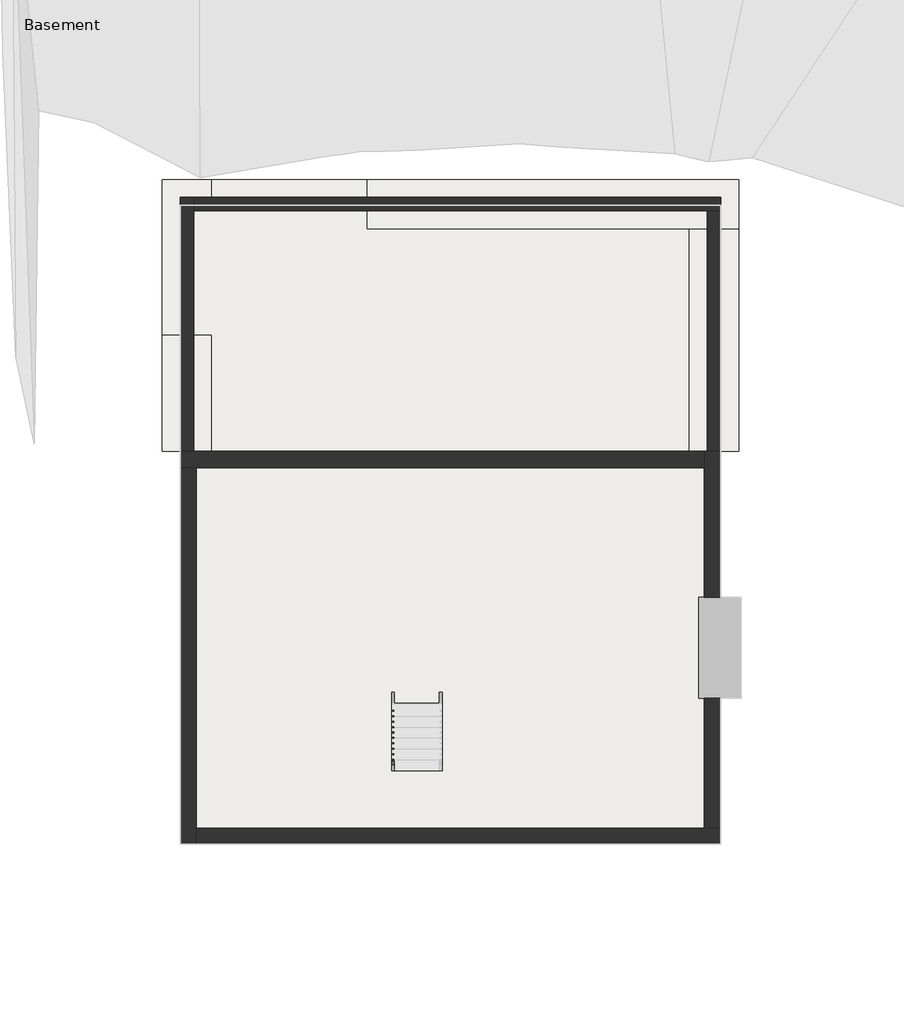
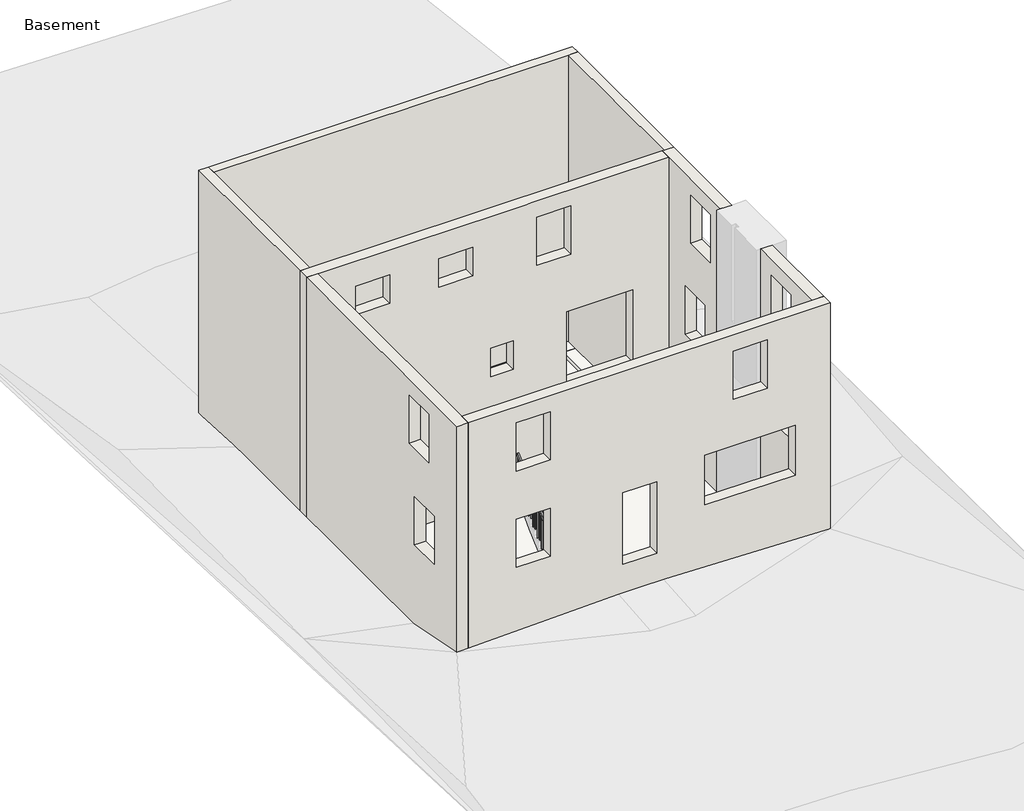
# One storey, part 1 of 2: 8 walls, 3 footings, 2 slabs, 1 railing.
"""IFC4 building model written with IfcOpenShell, lengths in millimetres."""

from ifc_helpers import new_model, si_unit, frame, origin, place, context, project, spatial, polyline, outline, extrude, faceted_brep, element, save

model = new_model("IFC4")

# Units and contexts
model_context = context("Model", 3, world=origin())
ifc_project = project(units=[si_unit("LENGTHUNIT", "METRE", prefix="MILLI")], contexts=[model_context])

# Site, building, storey
site = spatial("IfcSite", under=ifc_project)
building = spatial("IfcBuilding", under=site)
storey = spatial("IfcBuildingStorey", under=building, Name="Basement", Elevation=-2667.0)

# Footings
placement = place(None, origin())
element("IfcFooting", 1, ObjectType="Bearing Footing - 36\" x 12\"", at=placement, inside=storey, context=model_context, shape_type="Brep", body=[
    faceted_brep([(-5404.9803068, 3152.0888758, -2667.0), (-6319.3803068, 3152.0888758, -2667.0), (-6319.3803068, 3152.0888758, -2971.8), (-5404.9803068, 3152.0888758, -2971.8), (-6319.3803068, 5311.0888758, -2667.0), (-5404.9803068, 5311.0888758, -2667.0), (-5404.9803068, 5311.0888758, -2971.8), (-6319.3803068, 5311.0888758, -2971.8)], [[[0, 1, 2, 3]], [[4, 5, 6, 7]], [[0, 5, 4, 1]], [[2, 1, 4, 7]], [[3, 2, 7, 6]], [[0, 3, 6, 5]]]),
    faceted_brep([(-5404.9803068, 5311.0888758, -3124.2), (-6319.3803068, 5311.0888758, -3124.2), (-6319.3803068, 5311.0888758, -3429.0), (-5404.9803068, 5311.0888758, -3429.0), (-5404.9803068, 7292.2888758, -3124.2), (-5404.9803068, 8206.6888758, -3124.2), (-6319.3803068, 8206.6888758, -3124.2), (-6319.3803068, 8206.6888758, -3429.0), (-5404.9803068, 8206.6888758, -3429.0), (-5404.9803068, 7292.2888758, -3429.0)], [[[0, 1, 2, 3]], [[0, 4, 5, 6, 1]], [[2, 1, 6, 7]], [[3, 2, 7, 8, 9]], [[0, 3, 9, 8, 5, 4]], [[6, 5, 8, 7]]]),
])
element("IfcFooting", 2, ObjectType="Bearing Footing - 36\" x 12\"", at=placement, inside=storey, context=model_context, shape_type="Brep", body=[
    faceted_brep([(-2509.3803068, 8206.6888758, -3429.0), (-2509.3803068, 8206.6888758, -3124.2), (-2509.3803068, 7292.2888758, -3124.2), (-2509.3803068, 7292.2888758, -3429.0), (-5404.9803068, 8206.6888758, -3124.2), (-5404.9803068, 7292.2888758, -3124.2), (-5404.9803068, 8206.6888758, -3429.0), (-5404.9803068, 7292.2888758, -3429.0)], [[[0, 1, 2, 3]], [[2, 1, 4, 5]], [[1, 0, 6, 4]], [[0, 3, 7, 6]], [[3, 2, 5, 7]], [[5, 4, 6, 7]]]),
    faceted_brep([(-2509.3803068, 8206.6888758, -2667.0), (-2509.3803068, 8206.6888758, -2971.8), (-2509.3803068, 7292.2888758, -2971.8), (-2509.3803068, 7292.2888758, -2667.0), (4399.4196932, 8206.6888758, -2667.0), (3485.0196932, 7292.2888758, -2667.0), (4399.4196932, 7292.2888758, -2667.0), (4399.4196932, 8206.6888758, -2971.8), (4399.4196932, 7292.2888758, -2971.8), (3485.0196932, 7292.2888758, -2971.8)], [[[0, 1, 2, 3]], [[4, 0, 3, 5, 6]], [[1, 0, 4, 7]], [[2, 1, 7, 8, 9]], [[3, 2, 9, 8, 6, 5]], [[4, 6, 8, 7]]]),
])
element("IfcFooting", 3, ObjectType="Bearing Footing - 36\" x 12\"", at=placement, inside=storey, context=model_context, shape_type="SweptSolid", body=[
    extrude(outline(polyline([(4399.4196932, 3152.0888758), (3485.0196932, 3152.0888758), (3485.0196932, 7292.2888758), (4399.4196932, 7292.2888758), (4399.4196932, 3152.0888758)])), frame((0.0, 0.0, -2971.8), z_axis=(0.0, 0.0, 1.0), x_axis=(1.0, 0.0, 0.0)), (0.0, 0.0, 1.0), 304.8),
])

# Railing
element("IfcRailing", 4, ObjectType="Handrail - Rectangular", at=placement, inside=storey, context=model_context, shape_type="SweptSolid", body=[
    extrude(outline(polyline([(-2791.5111242, -1631.7331862), (-2791.5111242, -1562.1), (-149.9111242, 914.4), (-149.9111242, 844.7668138), (-2791.5111242, -1631.7331862)])), frame((-2052.1803068, 0.0, 0.0), z_axis=(1.0, 0.0, 0.0), x_axis=(0.0, 1.0, 0.0)), (0.0, 0.0, 1.0), 50.8),
    extrude(outline(polyline([(-241.9861242, 758.4465013), (-241.9861242, -190.5), (-261.0361242, -190.5), (-261.0361242, 740.5871263), (-241.9861242, 758.4465013)])), frame((-2036.3053068, 0.0, 0.0), z_axis=(1.0, 0.0, 0.0), x_axis=(0.0, 1.0, 0.0)), (0.0, 0.0, 1.0), 19.05),
    extrude(outline(polyline([(-343.5861242, 663.1965013), (-343.5861242, -190.5), (-362.6361242, -190.5), (-362.6361242, 645.3371263), (-343.5861242, 663.1965013)])), frame((-2036.3053068, 0.0, 0.0), z_axis=(1.0, 0.0, 0.0), x_axis=(0.0, 1.0, 0.0)), (0.0, 0.0, 1.0), 19.05),
    extrude(outline(polyline([(-445.1861242, 567.9465013), (-445.1861242, -381.0), (-464.2361242, -381.0), (-464.2361242, 550.0871263), (-445.1861242, 567.9465013)])), frame((-2036.3053068, 0.0, 0.0), z_axis=(1.0, 0.0, 0.0), x_axis=(0.0, 1.0, 0.0)), (0.0, 0.0, 1.0), 19.05),
    extrude(outline(polyline([(-546.7861242, 472.6965013), (-546.7861242, -381.0), (-565.8361242, -381.0), (-565.8361242, 454.8371263), (-546.7861242, 472.6965013)])), frame((-2036.3053068, 0.0, 0.0), z_axis=(1.0, 0.0, 0.0), x_axis=(0.0, 1.0, 0.0)), (0.0, 0.0, 1.0), 19.05),
    extrude(outline(polyline([(-648.3861242, 377.4465013), (-648.3861242, -571.5), (-667.4361242, -571.5), (-667.4361242, 359.5871263), (-648.3861242, 377.4465013)])), frame((-2036.3053068, 0.0, 0.0), z_axis=(1.0, 0.0, 0.0), x_axis=(0.0, 1.0, 0.0)), (0.0, 0.0, 1.0), 19.05),
    extrude(outline(polyline([(-749.9861242, 282.1965013), (-749.9861242, -571.5), (-769.0361242, -571.5), (-769.0361242, 264.3371263), (-749.9861242, 282.1965013)])), frame((-2036.3053068, 0.0, 0.0), z_axis=(1.0, 0.0, 0.0), x_axis=(0.0, 1.0, 0.0)), (0.0, 0.0, 1.0), 19.05),
    extrude(outline(polyline([(-851.5861242, 186.9465013), (-851.5861242, -762.0), (-870.6361242, -762.0), (-870.6361242, 169.0871263), (-851.5861242, 186.9465013)])), frame((-2036.3053068, 0.0, 0.0), z_axis=(1.0, 0.0, 0.0), x_axis=(0.0, 1.0, 0.0)), (0.0, 0.0, 1.0), 19.05),
    extrude(outline(polyline([(-953.1861242, 91.6965013), (-953.1861242, -762.0), (-972.2361242, -762.0), (-972.2361242, 73.8371263), (-953.1861242, 91.6965013)])), frame((-2036.3053068, 0.0, 0.0), z_axis=(1.0, 0.0, 0.0), x_axis=(0.0, 1.0, 0.0)), (0.0, 0.0, 1.0), 19.05),
    extrude(outline(polyline([(-1054.7861242, -3.5534987), (-1054.7861242, -952.5), (-1073.8361242, -952.5), (-1073.8361242, -21.4128737), (-1054.7861242, -3.5534987)])), frame((-2036.3053068, 0.0, 0.0), z_axis=(1.0, 0.0, 0.0), x_axis=(0.0, 1.0, 0.0)), (0.0, 0.0, 1.0), 19.05),
    extrude(outline(polyline([(-1156.3861242, -98.8034987), (-1156.3861242, -952.5), (-1175.4361242, -952.5), (-1175.4361242, -116.6628737), (-1156.3861242, -98.8034987)])), frame((-2036.3053068, 0.0, 0.0), z_axis=(1.0, 0.0, 0.0), x_axis=(0.0, 1.0, 0.0)), (0.0, 0.0, 1.0), 19.05),
    extrude(outline(polyline([(-1257.9861242, -194.0534987), (-1257.9861242, -1143.0), (-1277.0361242, -1143.0), (-1277.0361242, -211.9128737), (-1257.9861242, -194.0534987)])), frame((-2036.3053068, 0.0, 0.0), z_axis=(1.0, 0.0, 0.0), x_axis=(0.0, 1.0, 0.0)), (0.0, 0.0, 1.0), 19.05),
    extrude(outline(polyline([(-1359.5861242, -289.3034987), (-1359.5861242, -1143.0), (-1378.6361242, -1143.0), (-1378.6361242, -307.1628737), (-1359.5861242, -289.3034987)])), frame((-2036.3053068, 0.0, 0.0), z_axis=(1.0, 0.0, 0.0), x_axis=(0.0, 1.0, 0.0)), (0.0, 0.0, 1.0), 19.05),
    extrude(outline(polyline([(-1461.1861242, -384.5534987), (-1461.1861242, -1333.5), (-1480.2361242, -1333.5), (-1480.2361242, -402.4128737), (-1461.1861242, -384.5534987)])), frame((-2036.3053068, 0.0, 0.0), z_axis=(1.0, 0.0, 0.0), x_axis=(0.0, 1.0, 0.0)), (0.0, 0.0, 1.0), 19.05),
    extrude(outline(polyline([(-1562.7861242, -479.8034987), (-1562.7861242, -1333.5), (-1581.8361242, -1333.5), (-1581.8361242, -497.6628737), (-1562.7861242, -479.8034987)])), frame((-2036.3053068, 0.0, 0.0), z_axis=(1.0, 0.0, 0.0), x_axis=(0.0, 1.0, 0.0)), (0.0, 0.0, 1.0), 19.05),
    extrude(outline(polyline([(-1664.3861242, -575.0534987), (-1664.3861242, -1524.0), (-1683.4361242, -1524.0), (-1683.4361242, -592.9128737), (-1664.3861242, -575.0534987)])), frame((-2036.3053068, 0.0, 0.0), z_axis=(1.0, 0.0, 0.0), x_axis=(0.0, 1.0, 0.0)), (0.0, 0.0, 1.0), 19.05),
    extrude(outline(polyline([(-1765.9861242, -670.3034987), (-1765.9861242, -1524.0), (-1785.0361242, -1524.0), (-1785.0361242, -688.1628737), (-1765.9861242, -670.3034987)])), frame((-2036.3053068, 0.0, 0.0), z_axis=(1.0, 0.0, 0.0), x_axis=(0.0, 1.0, 0.0)), (0.0, 0.0, 1.0), 19.05),
    extrude(outline(polyline([(-1867.5861242, -765.5534987), (-1867.5861242, -1714.5), (-1886.6361242, -1714.5), (-1886.6361242, -783.4128737), (-1867.5861242, -765.5534987)])), frame((-2036.3053068, 0.0, 0.0), z_axis=(1.0, 0.0, 0.0), x_axis=(0.0, 1.0, 0.0)), (0.0, 0.0, 1.0), 19.05),
    extrude(outline(polyline([(-1969.1861242, -860.8034987), (-1969.1861242, -1714.5), (-1988.2361242, -1714.5), (-1988.2361242, -878.6628737), (-1969.1861242, -860.8034987)])), frame((-2036.3053068, 0.0, 0.0), z_axis=(1.0, 0.0, 0.0), x_axis=(0.0, 1.0, 0.0)), (0.0, 0.0, 1.0), 19.05),
    extrude(outline(polyline([(-2070.7861242, -956.0534987), (-2070.7861242, -1905.0), (-2089.8361242, -1905.0), (-2089.8361242, -973.9128737), (-2070.7861242, -956.0534987)])), frame((-2036.3053068, 0.0, 0.0), z_axis=(1.0, 0.0, 0.0), x_axis=(0.0, 1.0, 0.0)), (0.0, 0.0, 1.0), 19.05),
    extrude(outline(polyline([(-2172.3861242, -1051.3034987), (-2172.3861242, -1905.0), (-2191.4361242, -1905.0), (-2191.4361242, -1069.1628737), (-2172.3861242, -1051.3034987)])), frame((-2036.3053068, 0.0, 0.0), z_axis=(1.0, 0.0, 0.0), x_axis=(0.0, 1.0, 0.0)), (0.0, 0.0, 1.0), 19.05),
    extrude(outline(polyline([(-2273.9861242, -1146.5534987), (-2273.9861242, -2095.5), (-2293.0361242, -2095.5), (-2293.0361242, -1164.4128737), (-2273.9861242, -1146.5534987)])), frame((-2036.3053068, 0.0, 0.0), z_axis=(1.0, 0.0, 0.0), x_axis=(0.0, 1.0, 0.0)), (0.0, 0.0, 1.0), 19.05),
    extrude(outline(polyline([(-2375.5861242, -1241.8034987), (-2375.5861242, -2095.5), (-2394.6361242, -2095.5), (-2394.6361242, -1259.6628737), (-2375.5861242, -1241.8034987)])), frame((-2036.3053068, 0.0, 0.0), z_axis=(1.0, 0.0, 0.0), x_axis=(0.0, 1.0, 0.0)), (0.0, 0.0, 1.0), 19.05),
    extrude(outline(polyline([(-2477.1861242, -1337.0534987), (-2477.1861242, -2286.0), (-2496.2361242, -2286.0), (-2496.2361242, -1354.9128737), (-2477.1861242, -1337.0534987)])), frame((-2036.3053068, 0.0, 0.0), z_axis=(1.0, 0.0, 0.0), x_axis=(0.0, 1.0, 0.0)), (0.0, 0.0, 1.0), 19.05),
    extrude(outline(polyline([(-2578.7861242, -1432.3034987), (-2578.7861242, -2286.0), (-2597.8361242, -2286.0), (-2597.8361242, -1450.1628737), (-2578.7861242, -1432.3034987)])), frame((-2036.3053068, 0.0, 0.0), z_axis=(1.0, 0.0, 0.0), x_axis=(0.0, 1.0, 0.0)), (0.0, 0.0, 1.0), 19.05),
    extrude(outline(polyline([(-2680.3861242, -1527.5534987), (-2680.3861242, -2476.5), (-2699.4361242, -2476.5), (-2699.4361242, -1545.4128737), (-2680.3861242, -1527.5534987)])), frame((-2036.3053068, 0.0, 0.0), z_axis=(1.0, 0.0, 0.0), x_axis=(0.0, 1.0, 0.0)), (0.0, 0.0, 1.0), 19.05),
    extrude(outline(polyline([(-149.9111242, 844.7668138), (-149.9111242, -190.5), (-168.9611242, -190.5), (-168.9611242, 826.9074388), (-149.9111242, 844.7668138)])), frame((-2036.3053068, 0.0, 0.0), z_axis=(1.0, 0.0, 0.0), x_axis=(0.0, 1.0, 0.0)), (0.0, 0.0, 1.0), 19.05),
    extrude(outline(polyline([(-2772.4611242, -1613.8738112), (-2772.4611242, -2476.5), (-2791.5111242, -2476.5), (-2791.5111242, -1631.7331862), (-2772.4611242, -1613.8738112)])), frame((-2036.3053068, 0.0, 0.0), z_axis=(1.0, 0.0, 0.0), x_axis=(0.0, 1.0, 0.0)), (0.0, 0.0, 1.0), 19.05),
])

# Slabs
element("IfcSlab", 5, ObjectType="Pad 1", at=placement, inside=storey, context=model_context, shape_type="SweptSolid", body=[
    extrude(outline(polyline([(4069.2196932, 434.2888758), (4450.2196932, 434.2888758), (4450.2196932, -1445.3111242), (4069.2196932, -1445.3111242), (4069.2196932, -4163.1111242), (-5989.1803068, -4163.1111242), (-5989.1803068, 3152.0888758), (4069.2196932, 3152.0888758), (4069.2196932, 434.2888758)])), frame((0.0, 0.0, -3073.4), z_axis=(0.0, 0.0, 1.0), x_axis=(1.0, 0.0, 0.0)), (0.0, 0.0, 1.0), 304.8),
])
element("IfcSlab", 6, ObjectType="Pad 1", at=placement, inside=storey, context=model_context, shape_type="SweptSolid", body=[
    extrude(outline(polyline([(-5989.1803068, 7724.0888758), (4069.2196932, 7724.0888758), (4069.2196932, 3152.0888758), (-5989.1803068, 3152.0888758), (-5989.1803068, 7724.0888758)])), frame((0.0, 0.0, -3073.4), z_axis=(0.0, 0.0, 1.0), x_axis=(1.0, 0.0, 0.0)), (0.0, 0.0, 1.0), 304.8),
])

# Walls
element("IfcWall", 7, ObjectType="Generic - 10\"", at=placement, inside=storey, context=model_context, shape_type="Brep", body=[
    faceted_brep([(-5735.1803068, 3152.0888758, -2667.0), (-5735.1803068, 5311.0888758, -2667.0), (-5735.1803068, 5311.0888758, -3124.2), (-5735.1803068, 7622.4888758, -3124.2), (-5735.1803068, 7876.4888758, -3124.2), (-5735.1803068, 7876.4888758, 5486.4), (-5735.1803068, 7622.4888758, 5486.4), (-5735.1803068, 3152.0888758, 5486.4), (-5989.1803068, 3152.0888758, -2667.0), (-5989.1803068, 3152.0888758, 5486.4), (-5989.1803068, 7876.4888758, 5486.4), (-5989.1803068, 7876.4888758, -3124.2), (-5989.1803068, 5311.0888758, -3124.2), (-5989.1803068, 5311.0888758, -2667.0)], [[[0, 1, 2, 3, 4, 5, 6, 7]], [[8, 9, 10, 11, 12, 13]], [[1, 0, 8, 13]], [[2, 1, 13, 12]], [[4, 3, 2, 12, 11]], [[7, 6, 5, 10, 9]], [[5, 4, 11, 10]], [[0, 7, 9, 8]]]),
])
element("IfcWall", 8, ObjectType="Generic - 10\"", at=placement, inside=storey, context=model_context, shape_type="Brep", body=[
    faceted_brep([(-5735.1803068, 7622.4888758, -3124.2), (-2509.3803068, 7622.4888758, -3124.2), (-2509.3803068, 7622.4888758, -2667.0), (3815.2196932, 7622.4888758, -2667.0), (4069.2196932, 7622.4888758, -2667.0), (4069.2196932, 7622.4888758, 5486.4), (3815.2196932, 7622.4888758, 5486.4), (-5735.1803068, 7622.4888758, 5486.4), (-5735.1803068, 7876.4888758, -3124.2), (-5735.1803068, 7876.4888758, 5486.4), (4069.2196932, 7876.4888758, 5486.4), (4069.2196932, 7876.4888758, -2667.0), (-2509.3803068, 7876.4888758, -2667.0), (-2509.3803068, 7876.4888758, -3124.2)], [[[0, 1, 2, 3, 4, 5, 6, 7]], [[8, 9, 10, 11, 12, 13]], [[1, 0, 8, 13]], [[2, 1, 13, 12]], [[4, 3, 2, 12, 11]], [[7, 6, 5, 10, 9]], [[5, 4, 11, 10]], [[0, 7, 9, 8]]]),
])
element("IfcWall", 9, ObjectType="Generic - 10\"", at=placement, inside=storey, context=model_context, shape_type="SweptSolid", body=[
    extrude(outline(polyline([(3815.2196932, 3152.0888758), (3815.2196932, 7622.4888758), (4069.2196932, 7622.4888758), (4069.2196932, 3152.0888758), (3815.2196932, 3152.0888758)])), frame((0.0, 0.0, -2667.0), z_axis=(0.0, 0.0, 1.0), x_axis=(1.0, 0.0, 0.0)), (0.0, 0.0, 1.0), 8153.4),
])
element("IfcWall", 10, ObjectType="Generic - 12\"", at=placement, inside=storey, context=model_context, shape_type="Brep", body=[
    faceted_brep([(-5989.1803068, 2847.2888758, -2667.0), (-5684.3803068, 2847.2888758, -2667.0), (3764.4196932, 2847.2888758, -2667.0), (3764.4196932, 2847.2888758, 5486.4), (56.0196932, 2847.2888758, 5486.4), (-70.9803068, 2847.2888758, 5486.4), (-680.5803068, 2847.2888758, 5486.4), (-807.5803068, 2847.2888758, 5486.4), (-3169.7803068, 2847.2888758, 5486.4), (-3296.7803068, 2847.2888758, 5486.4), (-5684.3803068, 2847.2888758, 5486.4), (-5989.1803068, 2847.2888758, 5486.4), (1021.2196932, 2847.2888758, 0.0), (1021.2196932, 2847.2888758, 2057.4), (2799.2196932, 2847.2888758, 2057.4), (2799.2196932, 2847.2888758, 0.0), (-4160.3803068, 2847.2888758, 0.0), (-5023.9803068, 2847.2888758, 0.0), (-5023.9803068, 2847.2888758, 2032.0), (-4160.3803068, 2847.2888758, 2032.0), (-1036.1803068, 2847.2888758, 914.4), (-1036.1803068, 2847.2888758, 1727.2), (-426.5803068, 2847.2888758, 1727.2), (-426.5803068, 2847.2888758, 914.4), (-3919.0803068, 2847.2888758, 914.4), (-3919.0803068, 2847.2888758, 1727.2), (-3004.6803068, 2847.2888758, 1727.2), (-3004.6803068, 2847.2888758, 914.4), (208.4196932, 2847.2888758, 3657.6), (208.4196932, 2847.2888758, 5029.2), (1122.8196932, 2847.2888758, 5029.2), (1122.8196932, 2847.2888758, 3657.6), (-2433.1803068, 2847.2888758, 3962.4), (-2433.1803068, 2847.2888758, 4775.2), (-1518.7803068, 2847.2888758, 4775.2), (-1518.7803068, 2847.2888758, 3962.4), (-4668.3803068, 2847.2888758, 3962.4), (-4668.3803068, 2847.2888758, 4775.2), (-3753.9803068, 2847.2888758, 4775.2), (-3753.9803068, 2847.2888758, 3962.4), (3764.4196932, 3152.0888758, -2667.0), (-5989.1803068, 3152.0888758, -2667.0), (-5989.1803068, 3152.0888758, 5486.4), (3764.4196932, 3152.0888758, 5486.4), (1021.2196932, 3152.0888758, 2057.4), (1021.2196932, 3152.0888758, 0.0), (2799.2196932, 3152.0888758, 0.0), (2799.2196932, 3152.0888758, 2057.4), (-5023.9803068, 3152.0888758, 0.0), (-4160.3803068, 3152.0888758, 0.0), (-4160.3803068, 3152.0888758, 2032.0), (-5023.9803068, 3152.0888758, 2032.0), (-1036.1803068, 3152.0888758, 1727.2), (-1036.1803068, 3152.0888758, 914.4), (-426.5803068, 3152.0888758, 914.4), (-426.5803068, 3152.0888758, 1727.2), (-3919.0803068, 3152.0888758, 1727.2), (-3919.0803068, 3152.0888758, 914.4), (-3004.6803068, 3152.0888758, 914.4), (-3004.6803068, 3152.0888758, 1727.2), (208.4196932, 3152.0888758, 5029.2), (208.4196932, 3152.0888758, 3657.6), (1122.8196932, 3152.0888758, 3657.6), (1122.8196932, 3152.0888758, 5029.2), (-2433.1803068, 3152.0888758, 4775.2), (-2433.1803068, 3152.0888758, 3962.4), (-1518.7803068, 3152.0888758, 3962.4), (-1518.7803068, 3152.0888758, 4775.2), (-4668.3803068, 3152.0888758, 4775.2), (-4668.3803068, 3152.0888758, 3962.4), (-3753.9803068, 3152.0888758, 3962.4), (-3753.9803068, 3152.0888758, 4775.2)], [[[0, 1, 2, 3, 4, 5, 6, 7, 8, 9, 10, 11], [12, 13, 14, 15], [16, 17, 18, 19], [20, 21, 22, 23], [24, 25, 26, 27], [28, 29, 30, 31], [32, 33, 34, 35], [36, 37, 38, 39]], [[40, 41, 42, 43], [44, 45, 46, 47], [48, 49, 50, 51], [52, 53, 54, 55], [56, 57, 58, 59], [60, 61, 62, 63], [64, 65, 66, 67], [68, 69, 70, 71]], [[2, 1, 0, 41, 40]], [[11, 10, 9, 8, 7, 6, 5, 4, 3, 43, 42]], [[0, 11, 42, 41]], [[3, 2, 40, 43]], [[44, 13, 12, 45]], [[13, 44, 47, 14]], [[14, 47, 46, 15]], [[45, 12, 15, 46]], [[17, 16, 49, 48]], [[18, 17, 48, 51]], [[19, 18, 51, 50]], [[16, 19, 50, 49]], [[53, 52, 21, 20]], [[54, 53, 20, 23]], [[55, 54, 23, 22]], [[52, 55, 22, 21]], [[57, 56, 25, 24]], [[58, 57, 24, 27]], [[59, 58, 27, 26]], [[56, 59, 26, 25]], [[29, 28, 61, 60]], [[28, 31, 62, 61]], [[31, 30, 63, 62]], [[30, 29, 60, 63]], [[33, 32, 65, 64]], [[32, 35, 66, 65]], [[35, 34, 67, 66]], [[34, 33, 64, 67]], [[68, 37, 36, 69]], [[69, 36, 39, 70]], [[70, 39, 38, 71]], [[37, 68, 71, 38]]]),
])
element("IfcWall", 11, ObjectType="Generic - 12\"", at=placement, inside=storey, context=model_context, shape_type="Brep", body=[
    faceted_brep([(-5684.3803068, -4163.1111242, -2667.0), (-5684.3803068, -3858.3111242, -2667.0), (-5684.3803068, 2847.2888758, -2667.0), (-5684.3803068, 2847.2888758, 5486.4), (-5684.3803068, 1450.2888758, 5486.4), (-5684.3803068, 1323.2888758, 5486.4), (-5684.3803068, -3858.3111242, 5486.4), (-5684.3803068, -4163.1111242, 5486.4), (-5684.3803068, -3096.3111242, 914.4), (-5684.3803068, -3096.3111242, 2286.0), (-5684.3803068, -2181.9111242, 2286.0), (-5684.3803068, -2181.9111242, 914.4), (-5684.3803068, -2842.3111242, 3657.6), (-5684.3803068, -2842.3111242, 5029.2), (-5684.3803068, -1927.9111242, 5029.2), (-5684.3803068, -1927.9111242, 3657.6), (-5989.1803068, 2847.2888758, -2667.0), (-5989.1803068, -4163.1111242, -2667.0), (-5989.1803068, -4163.1111242, 5486.4), (-5989.1803068, 2847.2888758, 5486.4), (-5989.1803068, -3096.3111242, 2286.0), (-5989.1803068, -3096.3111242, 914.4), (-5989.1803068, -2181.9111242, 914.4), (-5989.1803068, -2181.9111242, 2286.0), (-5989.1803068, -2842.3111242, 5029.2), (-5989.1803068, -2842.3111242, 3657.6), (-5989.1803068, -1927.9111242, 3657.6), (-5989.1803068, -1927.9111242, 5029.2)], [[[0, 1, 2, 3, 4, 5, 6, 7], [8, 9, 10, 11], [12, 13, 14, 15]], [[16, 17, 18, 19], [20, 21, 22, 23], [24, 25, 26, 27]], [[2, 1, 0, 17, 16]], [[7, 6, 5, 4, 3, 19, 18]], [[0, 7, 18, 17]], [[3, 2, 16, 19]], [[21, 20, 9, 8]], [[22, 21, 8, 11]], [[23, 22, 11, 10]], [[20, 23, 10, 9]], [[24, 13, 12, 25]], [[25, 12, 15, 26]], [[26, 15, 14, 27]], [[13, 24, 27, 14]]]),
])
element("IfcWall", 12, ObjectType="Generic - 12\"", at=placement, inside=storey, context=model_context, shape_type="Brep", body=[
    faceted_brep([(4069.2196932, -3858.3111242, -2667.0), (3764.4196932, -3858.3111242, -2667.0), (-5684.3803068, -3858.3111242, -2667.0), (-5684.3803068, -3858.3111242, 5486.4), (-2179.1803068, -3858.3111242, 5486.4), (-2052.1803068, -3858.3111242, 5486.4), (-807.5803068, -3858.3111242, 5486.4), (-680.5803068, -3858.3111242, 5486.4), (-70.9803068, -3858.3111242, 5486.4), (56.0196932, -3858.3111242, 5486.4), (3764.4196932, -3858.3111242, 5486.4), (4069.2196932, -3858.3111242, 5486.4), (-1518.7803068, -3858.3111242, 0.0), (-604.3803068, -3858.3111242, 0.0), (-604.3803068, -3858.3111242, 2032.0), (-1518.7803068, -3858.3111242, 2032.0), (-3474.5803068, -3858.3111242, 914.4), (-3474.5803068, -3858.3111242, 2286.0), (-4388.9803068, -3858.3111242, 2286.0), (-4388.9803068, -3858.3111242, 914.4), (2367.4196932, -3858.3111242, 3657.6), (2367.4196932, -3858.3111242, 5029.2), (1453.0196932, -3858.3111242, 5029.2), (1453.0196932, -3858.3111242, 3657.6), (-3474.5803068, -3858.3111242, 3657.6), (-3474.5803068, -3858.3111242, 5029.2), (-4388.9803068, -3858.3111242, 5029.2), (-4388.9803068, -3858.3111242, 3657.6), (3129.4196932, -3858.3111242, 2336.8), (691.0196932, -3858.3111242, 2336.8), (691.0196932, -3858.3111242, 914.4), (3129.4196932, -3858.3111242, 914.4), (-5684.3803068, -4163.1111242, -2667.0), (4069.2196932, -4163.1111242, -2667.0), (4069.2196932, -4163.1111242, 5486.4), (-5684.3803068, -4163.1111242, 5486.4), (-604.3803068, -4163.1111242, 0.0), (-1518.7803068, -4163.1111242, 0.0), (-1518.7803068, -4163.1111242, 2032.0), (-604.3803068, -4163.1111242, 2032.0), (-3474.5803068, -4163.1111242, 2286.0), (-3474.5803068, -4163.1111242, 914.4), (-4388.9803068, -4163.1111242, 914.4), (-4388.9803068, -4163.1111242, 2286.0), (2367.4196932, -4163.1111242, 5029.2), (2367.4196932, -4163.1111242, 3657.6), (1453.0196932, -4163.1111242, 3657.6), (1453.0196932, -4163.1111242, 5029.2), (-3474.5803068, -4163.1111242, 5029.2), (-3474.5803068, -4163.1111242, 3657.6), (-4388.9803068, -4163.1111242, 3657.6), (-4388.9803068, -4163.1111242, 5029.2), (3129.4196932, -4163.1111242, 914.4), (691.0196932, -4163.1111242, 914.4), (691.0196932, -4163.1111242, 2336.8), (3129.4196932, -4163.1111242, 2336.8)], [[[0, 1, 2, 3, 4, 5, 6, 7, 8, 9, 10, 11], [12, 13, 14, 15], [16, 17, 18, 19], [20, 21, 22, 23], [24, 25, 26, 27], [28, 29, 30, 31]], [[32, 33, 34, 35], [36, 37, 38, 39], [40, 41, 42, 43], [44, 45, 46, 47], [48, 49, 50, 51], [52, 53, 54, 55]], [[2, 1, 0, 33, 32]], [[11, 10, 9, 8, 7, 6, 5, 4, 3, 35, 34]], [[0, 11, 34, 33]], [[3, 2, 32, 35]], [[37, 36, 13, 12]], [[38, 37, 12, 15]], [[39, 38, 15, 14]], [[36, 39, 14, 13]], [[41, 40, 17, 16]], [[42, 41, 16, 19]], [[43, 42, 19, 18]], [[40, 43, 18, 17]], [[30, 53, 52, 31]], [[54, 29, 28, 55]], [[29, 54, 53, 30]], [[31, 52, 55, 28]], [[21, 20, 45, 44]], [[20, 23, 46, 45]], [[23, 22, 47, 46]], [[22, 21, 44, 47]], [[25, 24, 49, 48]], [[24, 27, 50, 49]], [[27, 26, 51, 50]], [[26, 25, 48, 51]]]),
])
element("IfcWall", 13, ObjectType="Generic - 12\"", at=placement, inside=storey, context=model_context, shape_type="Brep", body=[
    faceted_brep([(3764.4196932, 3152.0888758, -2667.0), (3764.4196932, 2847.2888758, -2667.0), (3764.4196932, 434.2888758, -2667.0), (3764.4196932, 434.2888758, 5486.4), (3764.4196932, 2847.2888758, 5486.4), (3764.4196932, 3152.0888758, 5486.4), (3764.4196932, 2085.2888758, 914.4), (3764.4196932, 2085.2888758, 2286.0), (3764.4196932, 1170.8888758, 2286.0), (3764.4196932, 1170.8888758, 914.4), (3764.4196932, 1831.2888758, 3657.6), (3764.4196932, 1831.2888758, 5029.2), (3764.4196932, 916.8888758, 5029.2), (3764.4196932, 916.8888758, 3657.6), (4069.2196932, 434.2888758, -2667.0), (4069.2196932, 3152.0888758, -2667.0), (4069.2196932, 3152.0888758, 5486.4), (4069.2196932, 434.2888758, 5486.4), (4069.2196932, 2085.2888758, 2286.0), (4069.2196932, 2085.2888758, 914.4), (4069.2196932, 1170.8888758, 914.4), (4069.2196932, 1170.8888758, 2286.0), (4069.2196932, 1831.2888758, 5029.2), (4069.2196932, 1831.2888758, 3657.6), (4069.2196932, 916.8888758, 3657.6), (4069.2196932, 916.8888758, 5029.2)], [[[0, 1, 2, 3, 4, 5], [6, 7, 8, 9], [10, 11, 12, 13]], [[14, 15, 16, 17], [18, 19, 20, 21], [22, 23, 24, 25]], [[2, 1, 0, 15, 14]], [[3, 2, 14, 17]], [[5, 4, 3, 17, 16]], [[0, 5, 16, 15]], [[19, 18, 7, 6]], [[20, 19, 6, 9]], [[21, 20, 9, 8]], [[18, 21, 8, 7]], [[22, 11, 10, 23]], [[23, 10, 13, 24]], [[24, 13, 12, 25]], [[11, 22, 25, 12]]]),
])
element("IfcWall", 14, ObjectType="Generic - 12\"", at=placement, inside=storey, context=model_context, shape_type="SweptSolid", body=[
    extrude(outline(polyline([(-1445.3111242, -2667.0), (-3858.3111242, -2667.0), (-3858.3111242, 5486.4), (-1445.3111242, 5486.4), (-1445.3111242, -2667.0)]), holes=[polyline([(-2181.9111242, 2286.0), (-3096.3111242, 2286.0), (-3096.3111242, 914.4), (-2181.9111242, 914.4), (-2181.9111242, 2286.0)]), polyline([(-1927.9111242, 3657.6), (-1927.9111242, 5029.2), (-2842.3111242, 5029.2), (-2842.3111242, 3657.6), (-1927.9111242, 3657.6)])]), frame((3764.4196932, 0.0, 0.0), z_axis=(1.0, 0.0, 0.0), x_axis=(0.0, 1.0, 0.0)), (0.0, 0.0, 1.0), 304.8),
])

save(model, "model.ifc")

# Revit data of these elements
# Project information
#   Organization Name = "G3B Press"
#   Organization Description = "Paul F. Aubin Cosulting Services, Inc."
#   Building Name = "Revit Essentials for Architecture"
#   Author = "Paul F. Aubin"
#   Author Website = "https://www.paulaubin.com"
#   Copyright = "Copyright © 2020 Paul F Aubin, all rights reserved"
#   Project Issue Date = "8/1/2020"
#   Project Status = "Design Development"
#   Client Name = "Vertical Circulation"
#   Project Address = "789 Main ST\nAnytown, IL 60000"
#   Project Name = "08 Residential_Complete"
#   Project Number = "2020.03A"
# Type "Bearing Footing - 36\" x 12\""
#   Assembly Code = "A1010110"
# Type "Handrail - Rectangular"
#   Assembly Code = "C2010400"
#   built-in parameter 1008612 = 0.0416667 (stored number, unit not read)
#   built-in parameter 1008611 = 0.0416667 (stored number, unit not read)
#   built-in parameter 1008609 = 0.333333 (stored number, unit not read)
#   built-in parameter 1008604 = 0.166667 (stored number, unit not read)
#   built-in parameter 1008603 = 0.166667 (stored number, unit not read)
#   Railing Height = 3' - 0"
#   built-in parameter 1008630 = 2
#   built-in parameter 1008610 = 2
#   built-in parameter 1008618 = Baluster - Square : 3/4"
# Type "Pad 1"
#   Layers, outside or top first: 1' - 0" no material (function 1)
# Type "Generic - 10\""
#   Assembly Code = "B2010"
#   Layers, outside or top first: 0' - 10" no material (function 1)
# Type "Generic - 12\""
#   Assembly Code = "B2010"
#   Layers, outside or top first: 1' - 0" no material (function 1)
# Element 1 (IfcFooting, "Bearing Footing - 36\" x 12\"")
#   Phase Created = New Construction
#   Materials on its faces: "Concrete, Cast-in-Place gray"
# Elements 2, 3 (IfcFooting, "Bearing Footing - 36\" x 12\"")
#   Comments = ""
#   Phase Created = New Construction
#   Materials on its faces: "Concrete, Cast-in-Place gray"
# Element 4 (IfcRailing, "Handrail - Rectangular")
#   Phase Created = Existing
# Elements 5, 6 (IfcSlab, "Pad 1")
#   built-in parameter 1012502 = -0.333333 (stored number, unit not read)
#   Phase Created = New Construction
# Elements 7, 8, 9 (IfcWall, "Generic - 10\"")
#   Top Offset = 0' - 0"
#   Base Offset = 0' - 0"
#   wall height = 26' - 9"
#   Phase Created = New Construction
#   Base Constraint = Basement
#   Top Constraint = Roof
#   Materials on its faces: "Default Wall"
# Elements 10, 11, 12, 13, 14 (IfcWall, "Generic - 12\"")
#   Top Offset = 0' - 0"
#   Base Offset = 0' - 0"
#   wall height = 26' - 9"
#   Phase Created = Existing
#   Base Constraint = Basement
#   Top Constraint = Roof
#   Materials on its faces: "Default Wall"
# Materials
#   "Concrete, Cast-in-Place gray": class "Concrete", colour RGB 192 192 192, transparency 0, Description = "Cast-in-place concrete", Cost = 0
#   "Default Wall": class "Miscellaneous", colour RGB 128 128 128, transparency 0, Cost = 0
